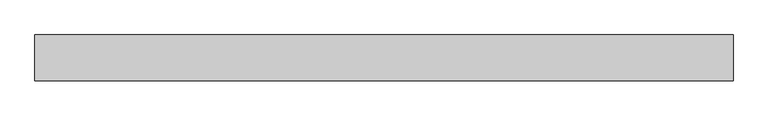
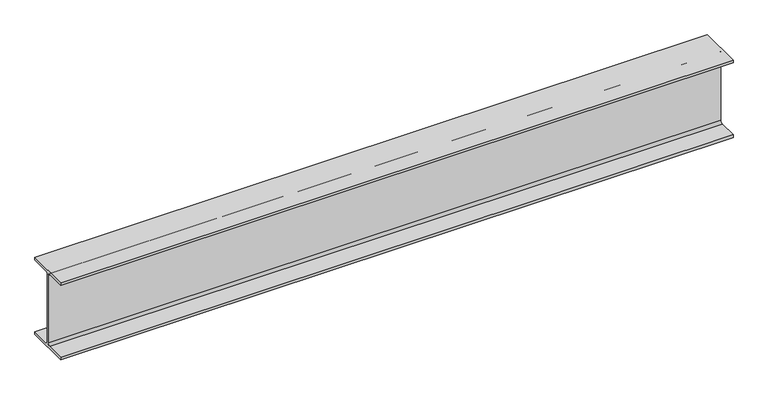
"""IFC4 building model written with IfcOpenShell, lengths in millimetres: beam geometry, Steel Beam_H-KSD3502 : H_SB_ASB_H-200x200x8x12."""

import ifcopenshell
import ifcopenshell.guid

model = None  # the IFC model being written
_history = None  # IfcOwnerHistory: only IFC2X3 demands one
_inside = {}  # id of a spatial element -> (the spatial element, [elements in it])
_under = {}  # id of a project, library or spatial element -> (it, [spatial elements below it])
_declared = {}  # id of a project -> (the project, [libraries it declares])
_typed = {}  # id of a type object -> (the type object, [elements of that type])
_made_of = {}  # id of a material, layer set ... -> (it, [elements and type objects made of it])


def new_model(schema):
    """Start an empty IFC model of exactly this schema.

    Asked for "IFC4X3", IfcOpenShell would pick the latest addendum, in which some entities
    have other attributes; the version numbers below select the first issue.
    IFC2X3 requires an IfcOwnerHistory on every rooted entity: one is made here for all.
    """
    global model, _history
    if schema == "IFC4X3":
        model = ifcopenshell.file(schema_version=(4, 3, 0, 0))
    else:
        model = ifcopenshell.file(schema=schema)
    _inside.clear()
    _under.clear()
    _declared.clear()
    _typed.clear()
    _made_of.clear()
    _history = None
    if model.schema == "IFC2X3":
        org = make("IfcOrganization", Name="unknown")
        user = make(
            "IfcPersonAndOrganization",
            ThePerson=make("IfcPerson", FamilyName="unknown"),
            TheOrganization=org,
        )
        app = make(
            "IfcApplication",
            ApplicationDeveloper=org,
            Version="unknown",
            ApplicationFullName="unknown",
            ApplicationIdentifier="unknown",
        )
        _history = make(
            "IfcOwnerHistory",
            OwningUser=user,
            OwningApplication=app,
            ChangeAction="ADDED",
            CreationDate=0,
        )
    return model


def make(cls, **values):
    """One entity of the class cls with the attributes given. An attribute that is None is left unset."""
    return model.create_entity(
        cls, **{name: value for name, value in values.items() if value is not None}
    )


def rooted(cls, **values):
    """An entity with a GlobalId (a new one), such as an element, a storey or a relation."""
    return make(cls, GlobalId=ifcopenshell.guid.new(), OwnerHistory=_history, **values)


def si_unit(unit_type, name, prefix=None):
    """IfcSIUnit, for example si_unit("LENGTHUNIT", "METRE", prefix="MILLI")."""
    return make("IfcSIUnit", UnitType=unit_type, Prefix=prefix, Name=name)


def assignment(units):
    """IfcUnitAssignment: the units of a project."""
    return None if units is None else make("IfcUnitAssignment", Units=units)


def point(xyz):
    """IfcCartesianPoint."""
    return None if xyz is None else make("IfcCartesianPoint", Coordinates=xyz)


def direction(xyz):
    """IfcDirection."""
    return None if xyz is None else make("IfcDirection", DirectionRatios=xyz)


def frame(location, z_axis=None, x_axis=None):
    """IfcAxis2Placement3D, a coordinate frame: its origin and axes. An axis left out is left unset."""
    return make(
        "IfcAxis2Placement3D",
        Location=point(location),
        Axis=direction(z_axis),
        RefDirection=direction(x_axis),
    )


def frame_2d(location, x_axis=None):
    """IfcAxis2Placement2D, a coordinate frame in the plane: its origin and x axis."""
    return make(
        "IfcAxis2Placement2D", Location=point(location), RefDirection=direction(x_axis)
    )


def origin():
    """The frame at (0, 0, 0) with its axes left unset."""
    return frame((0.0, 0.0, 0.0))


def place(relative_to, where):
    """IfcLocalPlacement: puts the frame where relative to a parent placement (None: the world)."""
    return make(
        "IfcLocalPlacement", PlacementRelTo=relative_to, RelativePlacement=where
    )


def context(
    kind, dimensions, precision=None, world=None, true_north=None, identifier=None
):
    """IfcGeometricRepresentationContext, for example the 3D "Model" context."""
    return make(
        "IfcGeometricRepresentationContext",
        ContextIdentifier=identifier,
        ContextType=kind,
        CoordinateSpaceDimension=dimensions,
        Precision=precision,
        WorldCoordinateSystem=world,
        TrueNorth=true_north,
    )


def project(units=None, contexts=None):
    """IfcProject with its units and contexts."""
    return rooted(
        "IfcProject",
        Name="project",
        RepresentationContexts=contexts,
        UnitsInContext=assignment(units),
    )


def spatial(cls, under=None, at=None, **own):
    """A site, building, storey or space (cls), placed at a placement, below another one or the project."""
    s = rooted(cls, ObjectPlacement=at, **own)
    if under is not None:
        _under.setdefault(under.id(), (under, []))[1].append(s)
    return s


def polyline(points):
    """IfcPolyline through the points."""
    return make("IfcPolyline", Points=[point(p) for p in points])


def circle_curve(where, radius):
    """IfcCircle in the frame where."""
    return make("IfcCircle", Position=where, Radius=radius)


def trimmed(basis, trim1, trim2, sense, master):
    """IfcTrimmedCurve: the piece of a basis curve between two trims."""
    return make(
        "IfcTrimmedCurve",
        BasisCurve=basis,
        Trim1=trim1,
        Trim2=trim2,
        SenseAgreement=sense,
        MasterRepresentation=master,
    )


def segment(curve, same_sense, transition):
    """IfcCompositeCurveSegment."""
    return make(
        "IfcCompositeCurveSegment",
        Transition=transition,
        SameSense=same_sense,
        ParentCurve=curve,
    )


def composite_curve(segments, self_intersect=None):
    """IfcCompositeCurve: segments joined end to end."""
    return make("IfcCompositeCurve", Segments=segments, SelfIntersect=self_intersect)


def outline(outer, holes=None, kind="AREA"):
    """IfcArbitraryClosedProfileDef: a profile drawn as a closed curve; with holes, ...WithVoids."""
    if holes is None:
        return make("IfcArbitraryClosedProfileDef", ProfileType=kind, OuterCurve=outer)
    return make(
        "IfcArbitraryProfileDefWithVoids",
        ProfileType=kind,
        OuterCurve=outer,
        InnerCurves=holes,
    )


def extrude(swept, where, along, depth):
    """IfcExtrudedAreaSolid: the profile swept, set in the frame where, extruded along a direction by depth."""
    return make(
        "IfcExtrudedAreaSolid",
        SweptArea=swept,
        Position=where,
        ExtrudedDirection=direction(along),
        Depth=depth,
    )


def shape(context_of_items, identifier, shape_type, items):
    """IfcShapeRepresentation: the items that make up one representation, for example the "Body"."""
    return make(
        "IfcShapeRepresentation",
        ContextOfItems=context_of_items,
        RepresentationIdentifier=identifier,
        RepresentationType=shape_type,
        Items=items,
    )


def source(mapping_origin, context_of_items, identifier, shape_type, items):
    """IfcRepresentationMap: a shape defined once, which mapped items show again and again."""
    return make(
        "IfcRepresentationMap",
        MappingOrigin=mapping_origin,
        MappedRepresentation=shape(context_of_items, identifier, shape_type, items),
    )


def transform(
    local_origin,
    x_axis=None,
    y_axis=None,
    z_axis=None,
    scale=None,
    scale2=None,
    scale3=None,
    uniform=True,
):
    """IfcCartesianTransformationOperator3D, or its non-uniform kind. x_axis, y_axis, z_axis: its Axis1, 2, 3."""
    if uniform:
        return make(
            "IfcCartesianTransformationOperator3D",
            Axis1=direction(x_axis),
            Axis2=direction(y_axis),
            LocalOrigin=point(local_origin),
            Scale=scale,
            Axis3=direction(z_axis),
        )
    return make(
        "IfcCartesianTransformationOperator3DnonUniform",
        Axis1=direction(x_axis),
        Axis2=direction(y_axis),
        LocalOrigin=point(local_origin),
        Scale=scale,
        Axis3=direction(z_axis),
        Scale2=scale2,
        Scale3=scale3,
    )


def mapped(mapping_source, mapping_target):
    """IfcMappedItem: shows the shape of a source again, moved by a transform."""
    return make(
        "IfcMappedItem", MappingSource=mapping_source, MappingTarget=mapping_target
    )


def made_of(thing, what):
    """Note that an element or type object is made of a material, layer set ...; save() writes the relation."""
    if what is not None:
        _made_of.setdefault(what.id(), (what, []))[1].append(thing)
    return thing


def element(
    cls,
    number,
    at=None,
    inside=None,
    cuts=None,
    type_object=None,
    material=None,
    context=None,
    identifier="Body",
    shape_type=None,
    held_by="IfcProductDefinitionShape",
    body=None,
    shapes=None,
    **own,
):
    """One element of the class cls, such as IfcWall. Its Tag is "e" and its number.

    at: its placement. inside: the storey or other place that contains it. cuts: it is an
    opening in that element (IfcRelVoidsElement). A single representation is given by context,
    identifier, shape_type and body (its items); several are given by shapes. held_by: the class
    of the entity that holds the representations. save() writes the other relations.
    """
    e = rooted(cls, Tag="e%d" % number, ObjectPlacement=at, **own)
    if body is not None:
        shapes = [shape(context, identifier, shape_type, body)]
    if shapes is not None:
        e.Representation = make(held_by, Representations=shapes)
    if inside is not None:
        _inside.setdefault(inside.id(), (inside, []))[1].append(e)
    if cuts is not None:
        rooted(
            "IfcRelVoidsElement", RelatingBuildingElement=cuts, RelatedOpeningElement=e
        )
    if type_object is not None:
        _typed.setdefault(type_object.id(), (type_object, []))[1].append(e)
    return made_of(e, material)


def aggregate(whole, parts):
    """IfcRelAggregates: a whole, such as a stair, and the parts it consists of."""
    return rooted("IfcRelAggregates", RelatingObject=whole, RelatedObjects=parts)


def save(model, path):
    """Write the relations noted so far, then the file.

    IfcRelAggregates (storeys below a building ...), IfcRelContainedInSpatialStructure (elements
    in a storey), IfcRelDefinesByType, IfcRelAssociatesMaterial and IfcRelDeclares: one each for
    every whole, place, type object, material and project.
    """
    for whole, parts in _under.values():
        aggregate(whole, parts)
    for where, things in _inside.values():
        rooted(
            "IfcRelContainedInSpatialStructure",
            RelatedElements=things,
            RelatingStructure=where,
        )
    for kind, things in _typed.values():
        rooted("IfcRelDefinesByType", RelatedObjects=things, RelatingType=kind)
    for what, things in _made_of.values():
        rooted("IfcRelAssociatesMaterial", RelatedObjects=things, RelatingMaterial=what)
    for by, libraries in _declared.values():
        rooted("IfcRelDeclares", RelatingContext=by, RelatedDefinitions=libraries)
    model.write(path)


def beam_1490ead7(model_context):
    return source(origin(), model_context, "Body", "SweptSolid", [
        extrude(outline(composite_curve([segment(polyline([(82.5, -141.5), (82.5, -151.7), (-82.5, -151.7), (-82.5, -141.5), (-11.9, -141.5)]), True, "CONTINUOUS"), segment(trimmed(circle_curve(frame_2d((-11.9, -132.6)), 8.9), [point((-11.9, -141.5))], [point((-3.0, -132.6))], True, "CARTESIAN"), True, "CONTINUOUS"), segment(polyline([(-3.0, -132.6), (-3.0, 132.6)]), True, "CONTINUOUS"), segment(trimmed(circle_curve(frame_2d((-11.9, 132.6)), 8.9), [point((-3.0, 132.6))], [point((-11.9, 141.5))], True, "CARTESIAN"), True, "CONTINUOUS"), segment(polyline([(-11.9, 141.5), (-82.5, 141.5), (-82.5, 151.7), (82.5, 151.7), (82.5, 141.5), (11.9, 141.5)]), True, "CONTINUOUS"), segment(trimmed(circle_curve(frame_2d((11.9, 132.6)), 8.9), [point((11.9, 141.5))], [point((3.0, 132.6))], True, "CARTESIAN"), True, "CONTINUOUS"), segment(polyline([(3.0, 132.6), (3.0, -132.6)]), True, "CONTINUOUS"), segment(trimmed(circle_curve(frame_2d((11.9, -132.6)), 8.9), [point((3.0, -132.6))], [point((11.9, -141.5))], True, "CARTESIAN"), True, "CONTINUOUS"), segment(polyline([(11.9, -141.5), (82.5, -141.5)]), True, "CONTINUOUS")], self_intersect=False)), frame((-1276.0000495, 0.0, 0.0), z_axis=(1.0, 0.0, 0.0), x_axis=(0.0, 1.0, 0.0)), (0.0, 0.0, 1.0), 2501.5236841),
    ])


if __name__ == "__main__":
    model = new_model("IFC4")
    model_context = context("Model", 3, world=origin())
    ifc_project = project(units=[si_unit("LENGTHUNIT", "METRE", prefix="MILLI")], contexts=[model_context])
    site = spatial("IfcSite", under=ifc_project)
    building = spatial("IfcBuilding", under=site)
    placement = place(None, origin())
    beam_shape = beam_1490ead7(model_context)
    element("IfcBeam", 1, ObjectType="Steel Beam_H-KSD3502 : H_SB_ASB_H-200x200x8x12", at=placement, inside=building, context=model_context, shape_type="MappedRepresentation", body=[
        mapped(beam_shape, transform((0.0, 0.0, 0.0), x_axis=(1.0, 0.0, 0.0), y_axis=(0.0, 1.0, 0.0), z_axis=(0.0, 0.0, 1.0))),
    ])
    save(model, "model.ifc")

# Revit data of these elements
# Type "Steel Beam_H-KSD3502 : H_SB_ASB_H-200x200x8x12"
#   Width = 20.0 cm
#   Web Thickness = 0.8 cm
#   Web Fillet = 1.3 cm
#   Warping Constant = 141376.0 cm⁶
#   Torsional Moment of Inertia = 26.2485 cm⁴
#   Torsional Modulus = 1.0 cm³
#   Section Area = 63.53 cm²
#   Plastic Modulus weak axis = 244.0 cm³
#   Plastic Modulus strong axis = 525.0 cm³
#   Perimeter = 1.16 m²/m
#   Nominal Weight = 49.90 kgf/m
#   Moment of Inertia weak axis = 1600.00 cm⁴
#   Moment of Inertia strong axis = 4720.00 cm⁴
#   Height = 20.0 cm
#   Flange Thickness = 1.2 cm
#   Elastic Modulus weak axis = 160.0 cm³
#   Elastic Modulus strong axis = 472.0 cm³
#   Centroid Vertical = 10.0 cm
#   Centroid Horizontal = 10.0 cm
#   Length [instance default] = 1.5240 m
#   Structural Material [instance default] = Steel, 45-345
#   Assembly Code = ""
# Element 1 (IfcBeam, "Steel Beam_H-KSD3502 : H_SB_ASB_H-200x200x8x12")
#   Structural Material = none
# Materials
#   "Steel, 45-345": class "Metal", colour RGB 189 187 185, transparency 0, Description = "Steel 345 MPa", Cost = 0
